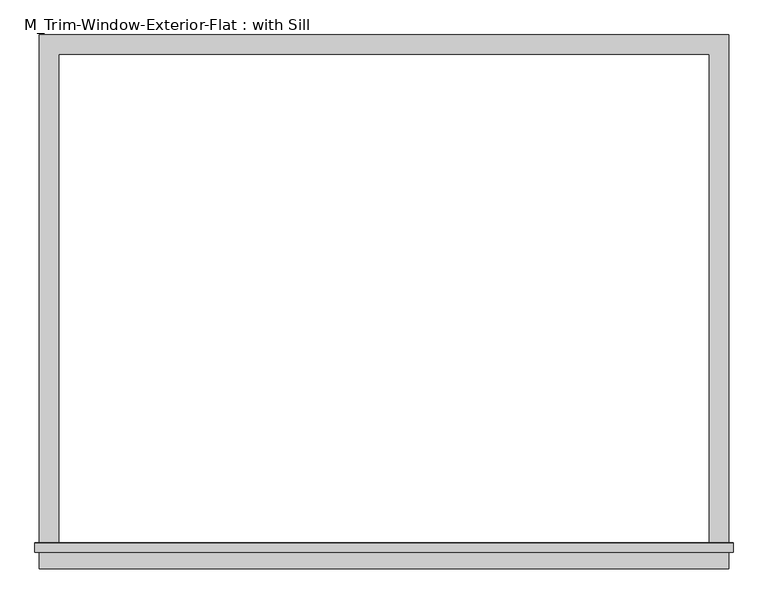
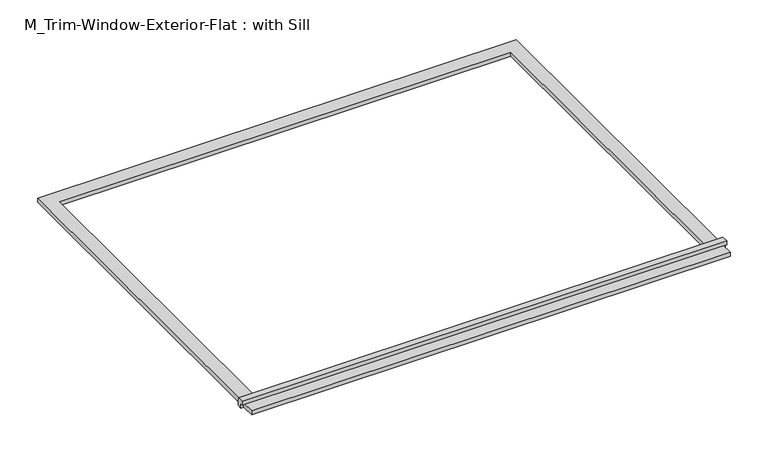
"""IFC4 building model written with IfcOpenShell, lengths in millimetres: proxy geometry, M_Trim-Window-Exterior-Flat : with Sill."""

from ifc_helpers import new_model, si_unit, frame, origin, origin_with_axes, place, context, project, spatial, polyline, outline, extrude, source, transform, mapped, element, save


def m_trim_window_exterior_flat_with_sill_41bea8b1(model_context):
    return source(origin(), model_context, "Body", "SweptSolid", [
        extrude(outline(polyline([(1060.0, -1520.4323709), (1060.0, -1580.4323709), (-1060.0, -1580.4323709), (-1060.0, -1520.4323709), (1060.0, -1520.4323709)])), origin_with_axes(), (0.0, 0.0, 1.0), 19.05),
        extrude(outline(polyline([(-1530.0, 38.1), (-1502.4580645, 38.1), (-1500.0, 19.05), (-1500.0, 0.0), (-1520.4323709, 0.0), (-1520.4323709, 19.05), (-1530.0, 19.05), (-1530.0, 38.1)])), frame((-1072.7, 0.0, 0.0), z_axis=(1.0, 0.0, 0.0), x_axis=(0.0, 1.0, 0.0)), (0.0, 0.0, 1.0), 2145.4),
        extrude(outline(polyline([(-1060.0, 60.0), (1060.0, 60.0), (1060.0, -1500.0), (1000.0, -1500.0), (1000.0, 0.0), (-1000.0, 0.0), (-1000.0, -1500.0), (-1060.0, -1500.0), (-1060.0, 60.0)])), origin_with_axes(), (0.0, 0.0, 1.0), 19.05),
    ])


if __name__ == "__main__":
    model = new_model("IFC4")
    model_context = context("Model", 3, world=origin())
    ifc_project = project(units=[si_unit("LENGTHUNIT", "METRE", prefix="MILLI")], contexts=[model_context])
    site = spatial("IfcSite", under=ifc_project)
    building = spatial("IfcBuilding", under=site)
    placement = place(None, origin())
    m_trim_window_exterior_flat_with_sill_shape = m_trim_window_exterior_flat_with_sill_41bea8b1(model_context)
    element("IfcBuildingElementProxy", 1, Name="M_Trim-Window-Exterior-Flat : with Sill", ObjectType="M_Trim-Window-Exterior-Flat : with Sill", at=placement, inside=building, context=model_context, shape_type="MappedRepresentation", body=[
        mapped(m_trim_window_exterior_flat_with_sill_shape, transform((0.0, 0.0, 0.0), x_axis=(1.0, 0.0, 0.0), y_axis=(0.0, 1.0, 0.0), z_axis=(0.0, 0.0, 1.0))),
    ])
    save(model, "model.ifc")

# Revit data of these elements
# Type "M_Trim-Window-Exterior-Flat : with Sill"
#   Trim Width = 60 mm
#   Trim Thickness_Picture Frame = 30 mm
#   Trim Thickness_with Sill = 19.05 mm
#   Sill Thickness = 30 mm
#   Opening Width [instance default] = 600 mm
#   Opening Height [instance default] = 900 mm
#   Default Elevation = 1200 mm
#   Sill = yes
#   Picture Frame = no
#   Trim Material [instance default] = none
# Element 1 (IfcBuildingElementProxy, "M_Trim-Window-Exterior-Flat : with Sill")
#   Opening Width = 2000 mm
#   Opening Height = 1500 mm
#   Trim Material = Clad - White
#   Materials on its faces: "Clad - White"
# Materials
#   "Clad - White": class "Wood", colour RGB 245 245 243, transparency 0, Cost = 0
